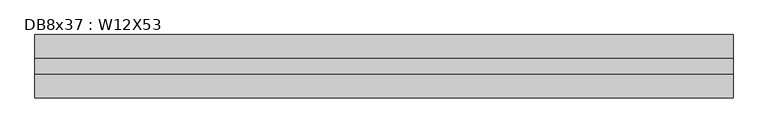
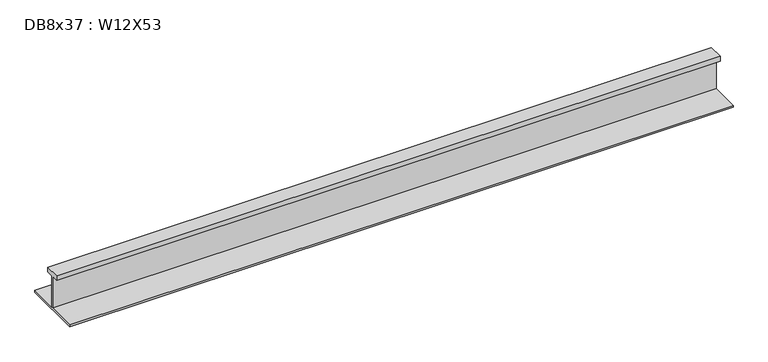
"""IFC4 building model written with IfcOpenShell, lengths in millimetres: beam geometry, DB8x37 : W12X53."""

from ifc_helpers import new_model, si_unit, frame, origin, place, context, project, spatial, polyline, outline, extrude, source, transform, mapped, element, save


def db8x37_w12x53_32495ae0(model_context):
    return source(origin(), model_context, "Body", "SweptSolid", [
        extrude(outline(polyline([(38.1, 145.415), (38.1, 120.015), (2.921, 120.015), (2.921, -48.4505), (152.4, -48.4505), (152.4, -58.1025), (-152.4, -58.1025), (-152.4, -48.4505), (-2.921, -48.4505), (-2.921, 120.015), (-38.1, 120.015), (-38.1, 145.415), (38.1, 145.415)])), frame((-1679.829, 0.0, 0.0), z_axis=(1.0, 0.0, 0.0), x_axis=(0.0, 1.0, 0.0)), (0.0, 0.0, 1.0), 3359.658),
    ])


if __name__ == "__main__":
    model = new_model("IFC4")
    model_context = context("Model", 3, world=origin())
    ifc_project = project(units=[si_unit("LENGTHUNIT", "METRE", prefix="MILLI")], contexts=[model_context])
    site = spatial("IfcSite", under=ifc_project)
    building = spatial("IfcBuilding", under=site)
    placement = place(None, origin())
    db8x37_w12x53_shape = db8x37_w12x53_32495ae0(model_context)
    element("IfcBeam", 1, ObjectType="DB8x37 : W12X53", at=placement, inside=building, context=model_context, shape_type="MappedRepresentation", body=[
        mapped(db8x37_w12x53_shape, transform((0.0, 0.0, 0.0), x_axis=(1.0, 0.0, 0.0), y_axis=(0.0, 1.0, 0.0), z_axis=(0.0, 0.0, 1.0))),
    ])
    save(model, "model.ifc")

# Revit data of these elements
# Type "DB8x37 : W12X53"
#   Assembly Code = "B10"
#   W = 53
#   Length [instance default] = 5' - 0"
#   bf = 0' - 10"
#   d = 1' - 0.1"
#   k = 0' - 1 3/8"
#   k2 = 0' - 0.8"
#   tf = 0' - 0.575"
#   tw = 0' - 0.345"
#   A = 0.108333 SF
#   Structural Material [instance default] = Steel ASTM A992
# Element 1 (IfcBeam, "DB8x37 : W12X53")
#   Materials on its faces: "Steel ASTM A992"
# Materials
#   "Steel ASTM A992": class "Metal", colour RGB 199 199 199, transparency 0, Description = "Structural steel 50ksi", Cost = 0
